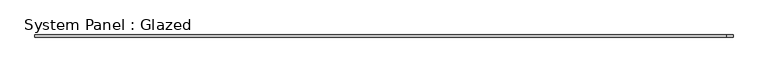
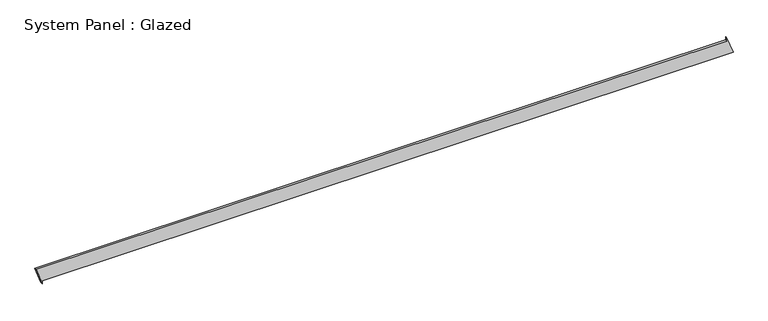
"""IFC4 building model written with IfcOpenShell, lengths in millimetres: plate geometry, System Panel : Glazed."""

import ifcopenshell
import ifcopenshell.guid

model = None  # the IFC model being written
_history = None  # IfcOwnerHistory: only IFC2X3 demands one
_inside = {}  # id of a spatial element -> (the spatial element, [elements in it])
_under = {}  # id of a project, library or spatial element -> (it, [spatial elements below it])
_declared = {}  # id of a project -> (the project, [libraries it declares])
_typed = {}  # id of a type object -> (the type object, [elements of that type])
_made_of = {}  # id of a material, layer set ... -> (it, [elements and type objects made of it])


def new_model(schema):
    """Start an empty IFC model of exactly this schema.

    Asked for "IFC4X3", IfcOpenShell would pick the latest addendum, in which some entities
    have other attributes; the version numbers below select the first issue.
    IFC2X3 requires an IfcOwnerHistory on every rooted entity: one is made here for all.
    """
    global model, _history
    if schema == "IFC4X3":
        model = ifcopenshell.file(schema_version=(4, 3, 0, 0))
    else:
        model = ifcopenshell.file(schema=schema)
    _inside.clear()
    _under.clear()
    _declared.clear()
    _typed.clear()
    _made_of.clear()
    _history = None
    if model.schema == "IFC2X3":
        org = make("IfcOrganization", Name="unknown")
        user = make(
            "IfcPersonAndOrganization",
            ThePerson=make("IfcPerson", FamilyName="unknown"),
            TheOrganization=org,
        )
        app = make(
            "IfcApplication",
            ApplicationDeveloper=org,
            Version="unknown",
            ApplicationFullName="unknown",
            ApplicationIdentifier="unknown",
        )
        _history = make(
            "IfcOwnerHistory",
            OwningUser=user,
            OwningApplication=app,
            ChangeAction="ADDED",
            CreationDate=0,
        )
    return model


def make(cls, **values):
    """One entity of the class cls with the attributes given. An attribute that is None is left unset."""
    return model.create_entity(
        cls, **{name: value for name, value in values.items() if value is not None}
    )


def rooted(cls, **values):
    """An entity with a GlobalId (a new one), such as an element, a storey or a relation."""
    return make(cls, GlobalId=ifcopenshell.guid.new(), OwnerHistory=_history, **values)


def si_unit(unit_type, name, prefix=None):
    """IfcSIUnit, for example si_unit("LENGTHUNIT", "METRE", prefix="MILLI")."""
    return make("IfcSIUnit", UnitType=unit_type, Prefix=prefix, Name=name)


def assignment(units):
    """IfcUnitAssignment: the units of a project."""
    return None if units is None else make("IfcUnitAssignment", Units=units)


def point(xyz):
    """IfcCartesianPoint."""
    return None if xyz is None else make("IfcCartesianPoint", Coordinates=xyz)


def direction(xyz):
    """IfcDirection."""
    return None if xyz is None else make("IfcDirection", DirectionRatios=xyz)


def frame(location, z_axis=None, x_axis=None):
    """IfcAxis2Placement3D, a coordinate frame: its origin and axes. An axis left out is left unset."""
    return make(
        "IfcAxis2Placement3D",
        Location=point(location),
        Axis=direction(z_axis),
        RefDirection=direction(x_axis),
    )


def origin():
    """The frame at (0, 0, 0) with its axes left unset."""
    return frame((0.0, 0.0, 0.0))


def place(relative_to, where):
    """IfcLocalPlacement: puts the frame where relative to a parent placement (None: the world)."""
    return make(
        "IfcLocalPlacement", PlacementRelTo=relative_to, RelativePlacement=where
    )


def context(
    kind, dimensions, precision=None, world=None, true_north=None, identifier=None
):
    """IfcGeometricRepresentationContext, for example the 3D "Model" context."""
    return make(
        "IfcGeometricRepresentationContext",
        ContextIdentifier=identifier,
        ContextType=kind,
        CoordinateSpaceDimension=dimensions,
        Precision=precision,
        WorldCoordinateSystem=world,
        TrueNorth=true_north,
    )


def project(units=None, contexts=None):
    """IfcProject with its units and contexts."""
    return rooted(
        "IfcProject",
        Name="project",
        RepresentationContexts=contexts,
        UnitsInContext=assignment(units),
    )


def spatial(cls, under=None, at=None, **own):
    """A site, building, storey or space (cls), placed at a placement, below another one or the project."""
    s = rooted(cls, ObjectPlacement=at, **own)
    if under is not None:
        _under.setdefault(under.id(), (under, []))[1].append(s)
    return s


def polyline(points):
    """IfcPolyline through the points."""
    return make("IfcPolyline", Points=[point(p) for p in points])


def outline(outer, holes=None, kind="AREA"):
    """IfcArbitraryClosedProfileDef: a profile drawn as a closed curve; with holes, ...WithVoids."""
    if holes is None:
        return make("IfcArbitraryClosedProfileDef", ProfileType=kind, OuterCurve=outer)
    return make(
        "IfcArbitraryProfileDefWithVoids",
        ProfileType=kind,
        OuterCurve=outer,
        InnerCurves=holes,
    )


def extrude(swept, where, along, depth):
    """IfcExtrudedAreaSolid: the profile swept, set in the frame where, extruded along a direction by depth."""
    return make(
        "IfcExtrudedAreaSolid",
        SweptArea=swept,
        Position=where,
        ExtrudedDirection=direction(along),
        Depth=depth,
    )


def shape(context_of_items, identifier, shape_type, items):
    """IfcShapeRepresentation: the items that make up one representation, for example the "Body"."""
    return make(
        "IfcShapeRepresentation",
        ContextOfItems=context_of_items,
        RepresentationIdentifier=identifier,
        RepresentationType=shape_type,
        Items=items,
    )


def source(mapping_origin, context_of_items, identifier, shape_type, items):
    """IfcRepresentationMap: a shape defined once, which mapped items show again and again."""
    return make(
        "IfcRepresentationMap",
        MappingOrigin=mapping_origin,
        MappedRepresentation=shape(context_of_items, identifier, shape_type, items),
    )


def transform(
    local_origin,
    x_axis=None,
    y_axis=None,
    z_axis=None,
    scale=None,
    scale2=None,
    scale3=None,
    uniform=True,
):
    """IfcCartesianTransformationOperator3D, or its non-uniform kind. x_axis, y_axis, z_axis: its Axis1, 2, 3."""
    if uniform:
        return make(
            "IfcCartesianTransformationOperator3D",
            Axis1=direction(x_axis),
            Axis2=direction(y_axis),
            LocalOrigin=point(local_origin),
            Scale=scale,
            Axis3=direction(z_axis),
        )
    return make(
        "IfcCartesianTransformationOperator3DnonUniform",
        Axis1=direction(x_axis),
        Axis2=direction(y_axis),
        LocalOrigin=point(local_origin),
        Scale=scale,
        Axis3=direction(z_axis),
        Scale2=scale2,
        Scale3=scale3,
    )


def mapped(mapping_source, mapping_target):
    """IfcMappedItem: shows the shape of a source again, moved by a transform."""
    return make(
        "IfcMappedItem", MappingSource=mapping_source, MappingTarget=mapping_target
    )


def made_of(thing, what):
    """Note that an element or type object is made of a material, layer set ...; save() writes the relation."""
    if what is not None:
        _made_of.setdefault(what.id(), (what, []))[1].append(thing)
    return thing


def element(
    cls,
    number,
    at=None,
    inside=None,
    cuts=None,
    type_object=None,
    material=None,
    context=None,
    identifier="Body",
    shape_type=None,
    held_by="IfcProductDefinitionShape",
    body=None,
    shapes=None,
    **own,
):
    """One element of the class cls, such as IfcWall. Its Tag is "e" and its number.

    at: its placement. inside: the storey or other place that contains it. cuts: it is an
    opening in that element (IfcRelVoidsElement). A single representation is given by context,
    identifier, shape_type and body (its items); several are given by shapes. held_by: the class
    of the entity that holds the representations. save() writes the other relations.
    """
    e = rooted(cls, Tag="e%d" % number, ObjectPlacement=at, **own)
    if body is not None:
        shapes = [shape(context, identifier, shape_type, body)]
    if shapes is not None:
        e.Representation = make(held_by, Representations=shapes)
    if inside is not None:
        _inside.setdefault(inside.id(), (inside, []))[1].append(e)
    if cuts is not None:
        rooted(
            "IfcRelVoidsElement", RelatingBuildingElement=cuts, RelatedOpeningElement=e
        )
    if type_object is not None:
        _typed.setdefault(type_object.id(), (type_object, []))[1].append(e)
    return made_of(e, material)


def aggregate(whole, parts):
    """IfcRelAggregates: a whole, such as a stair, and the parts it consists of."""
    return rooted("IfcRelAggregates", RelatingObject=whole, RelatedObjects=parts)


def save(model, path):
    """Write the relations noted so far, then the file.

    IfcRelAggregates (storeys below a building ...), IfcRelContainedInSpatialStructure (elements
    in a storey), IfcRelDefinesByType, IfcRelAssociatesMaterial and IfcRelDeclares: one each for
    every whole, place, type object, material and project.
    """
    for whole, parts in _under.values():
        aggregate(whole, parts)
    for where, things in _inside.values():
        rooted(
            "IfcRelContainedInSpatialStructure",
            RelatedElements=things,
            RelatingStructure=where,
        )
    for kind, things in _typed.values():
        rooted("IfcRelDefinesByType", RelatedObjects=things, RelatingType=kind)
    for what, things in _made_of.values():
        rooted("IfcRelAssociatesMaterial", RelatedObjects=things, RelatingMaterial=what)
    for by, libraries in _declared.values():
        rooted("IfcRelDeclares", RelatingContext=by, RelatedDefinitions=libraries)
    model.write(path)


def system_panel_glazed_eac3060f(model_context):
    return source(origin(), model_context, "Body", "SweptSolid", [
        extrude(outline(polyline([(0.0, -3956.878339), (35.3553391, -3956.878339), (35.3553391, 4027.1816216), (233.9801319, 3956.6725023), (198.6247928, 3956.6721138), (198.7125272, -4027.1816216), (0.0, -3956.878339)])), frame((0.0, -49.5, 0.0), z_axis=(0.0, 1.0, 0.0), x_axis=(0.0, 0.0, 1.0)), (0.0, 0.0, 1.0), 25.0),
    ])


if __name__ == "__main__":
    model = new_model("IFC4")
    model_context = context("Model", 3, world=origin())
    ifc_project = project(units=[si_unit("LENGTHUNIT", "METRE", prefix="MILLI")], contexts=[model_context])
    site = spatial("IfcSite", under=ifc_project)
    building = spatial("IfcBuilding", under=site)
    placement = place(None, origin())
    system_panel_glazed_shape = system_panel_glazed_eac3060f(model_context)
    element("IfcPlate", 1, ObjectType="System Panel : Glazed", at=placement, inside=building, context=model_context, shape_type="MappedRepresentation", body=[
        mapped(system_panel_glazed_shape, transform((0.0, 0.0, 0.0), x_axis=(1.0, 0.0, 0.0), y_axis=(0.0, 1.0, 0.0), z_axis=(0.0, 0.0, 1.0))),
    ])
    save(model, "model.ifc")

# Revit data of these elements
# Element 1 (IfcPlate, "System Panel : Glazed")
#   Materials on its faces: "Glass"
# Materials
#   "Glass": class "Glass", colour RGB 218 227 224, transparency 0.85, Description = "Soda Lime Glass", Cost = 0
